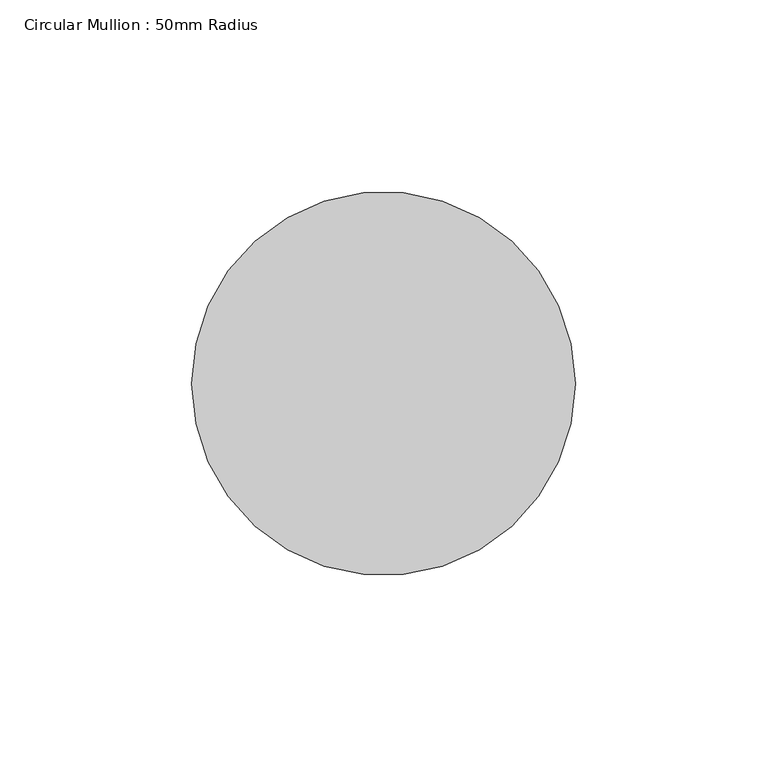
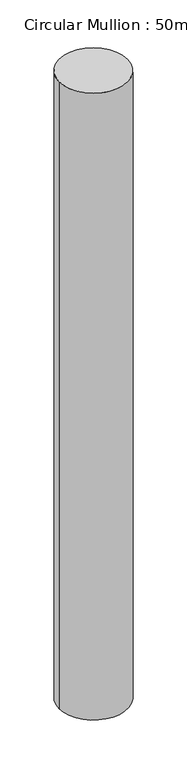
"""IFC4 building model written with IfcOpenShell, lengths in millimetres: member geometry, Circular Mullion : 50mm Radius."""

import ifcopenshell
import ifcopenshell.guid

model = None  # the IFC model being written
_history = None  # IfcOwnerHistory: only IFC2X3 demands one
_inside = {}  # id of a spatial element -> (the spatial element, [elements in it])
_under = {}  # id of a project, library or spatial element -> (it, [spatial elements below it])
_declared = {}  # id of a project -> (the project, [libraries it declares])
_typed = {}  # id of a type object -> (the type object, [elements of that type])
_made_of = {}  # id of a material, layer set ... -> (it, [elements and type objects made of it])


def new_model(schema):
    """Start an empty IFC model of exactly this schema.

    Asked for "IFC4X3", IfcOpenShell would pick the latest addendum, in which some entities
    have other attributes; the version numbers below select the first issue.
    IFC2X3 requires an IfcOwnerHistory on every rooted entity: one is made here for all.
    """
    global model, _history
    if schema == "IFC4X3":
        model = ifcopenshell.file(schema_version=(4, 3, 0, 0))
    else:
        model = ifcopenshell.file(schema=schema)
    _inside.clear()
    _under.clear()
    _declared.clear()
    _typed.clear()
    _made_of.clear()
    _history = None
    if model.schema == "IFC2X3":
        org = make("IfcOrganization", Name="unknown")
        user = make(
            "IfcPersonAndOrganization",
            ThePerson=make("IfcPerson", FamilyName="unknown"),
            TheOrganization=org,
        )
        app = make(
            "IfcApplication",
            ApplicationDeveloper=org,
            Version="unknown",
            ApplicationFullName="unknown",
            ApplicationIdentifier="unknown",
        )
        _history = make(
            "IfcOwnerHistory",
            OwningUser=user,
            OwningApplication=app,
            ChangeAction="ADDED",
            CreationDate=0,
        )
    return model


def make(cls, **values):
    """One entity of the class cls with the attributes given. An attribute that is None is left unset."""
    return model.create_entity(
        cls, **{name: value for name, value in values.items() if value is not None}
    )


def rooted(cls, **values):
    """An entity with a GlobalId (a new one), such as an element, a storey or a relation."""
    return make(cls, GlobalId=ifcopenshell.guid.new(), OwnerHistory=_history, **values)


def si_unit(unit_type, name, prefix=None):
    """IfcSIUnit, for example si_unit("LENGTHUNIT", "METRE", prefix="MILLI")."""
    return make("IfcSIUnit", UnitType=unit_type, Prefix=prefix, Name=name)


def assignment(units):
    """IfcUnitAssignment: the units of a project."""
    return None if units is None else make("IfcUnitAssignment", Units=units)


def point(xyz):
    """IfcCartesianPoint."""
    return None if xyz is None else make("IfcCartesianPoint", Coordinates=xyz)


def direction(xyz):
    """IfcDirection."""
    return None if xyz is None else make("IfcDirection", DirectionRatios=xyz)


def frame(location, z_axis=None, x_axis=None):
    """IfcAxis2Placement3D, a coordinate frame: its origin and axes. An axis left out is left unset."""
    return make(
        "IfcAxis2Placement3D",
        Location=point(location),
        Axis=direction(z_axis),
        RefDirection=direction(x_axis),
    )


def frame_2d(location, x_axis=None):
    """IfcAxis2Placement2D, a coordinate frame in the plane: its origin and x axis."""
    return make(
        "IfcAxis2Placement2D", Location=point(location), RefDirection=direction(x_axis)
    )


def origin():
    """The frame at (0, 0, 0) with its axes left unset."""
    return frame((0.0, 0.0, 0.0))


def origin_2d():
    """The frame at (0, 0) in the plane with its x axis left unset."""
    return frame_2d((0.0, 0.0))


def place(relative_to, where):
    """IfcLocalPlacement: puts the frame where relative to a parent placement (None: the world)."""
    return make(
        "IfcLocalPlacement", PlacementRelTo=relative_to, RelativePlacement=where
    )


def context(
    kind, dimensions, precision=None, world=None, true_north=None, identifier=None
):
    """IfcGeometricRepresentationContext, for example the 3D "Model" context."""
    return make(
        "IfcGeometricRepresentationContext",
        ContextIdentifier=identifier,
        ContextType=kind,
        CoordinateSpaceDimension=dimensions,
        Precision=precision,
        WorldCoordinateSystem=world,
        TrueNorth=true_north,
    )


def project(units=None, contexts=None):
    """IfcProject with its units and contexts."""
    return rooted(
        "IfcProject",
        Name="project",
        RepresentationContexts=contexts,
        UnitsInContext=assignment(units),
    )


def spatial(cls, under=None, at=None, **own):
    """A site, building, storey or space (cls), placed at a placement, below another one or the project."""
    s = rooted(cls, ObjectPlacement=at, **own)
    if under is not None:
        _under.setdefault(under.id(), (under, []))[1].append(s)
    return s


def circle_curve(where, radius):
    """IfcCircle in the frame where."""
    return make("IfcCircle", Position=where, Radius=radius)


def trimmed(basis, trim1, trim2, sense, master):
    """IfcTrimmedCurve: the piece of a basis curve between two trims."""
    return make(
        "IfcTrimmedCurve",
        BasisCurve=basis,
        Trim1=trim1,
        Trim2=trim2,
        SenseAgreement=sense,
        MasterRepresentation=master,
    )


def segment(curve, same_sense, transition):
    """IfcCompositeCurveSegment."""
    return make(
        "IfcCompositeCurveSegment",
        Transition=transition,
        SameSense=same_sense,
        ParentCurve=curve,
    )


def composite_curve(segments, self_intersect=None):
    """IfcCompositeCurve: segments joined end to end."""
    return make("IfcCompositeCurve", Segments=segments, SelfIntersect=self_intersect)


def outline(outer, holes=None, kind="AREA"):
    """IfcArbitraryClosedProfileDef: a profile drawn as a closed curve; with holes, ...WithVoids."""
    if holes is None:
        return make("IfcArbitraryClosedProfileDef", ProfileType=kind, OuterCurve=outer)
    return make(
        "IfcArbitraryProfileDefWithVoids",
        ProfileType=kind,
        OuterCurve=outer,
        InnerCurves=holes,
    )


def extrude(swept, where, along, depth):
    """IfcExtrudedAreaSolid: the profile swept, set in the frame where, extruded along a direction by depth."""
    return make(
        "IfcExtrudedAreaSolid",
        SweptArea=swept,
        Position=where,
        ExtrudedDirection=direction(along),
        Depth=depth,
    )


def shape(context_of_items, identifier, shape_type, items):
    """IfcShapeRepresentation: the items that make up one representation, for example the "Body"."""
    return make(
        "IfcShapeRepresentation",
        ContextOfItems=context_of_items,
        RepresentationIdentifier=identifier,
        RepresentationType=shape_type,
        Items=items,
    )


def source(mapping_origin, context_of_items, identifier, shape_type, items):
    """IfcRepresentationMap: a shape defined once, which mapped items show again and again."""
    return make(
        "IfcRepresentationMap",
        MappingOrigin=mapping_origin,
        MappedRepresentation=shape(context_of_items, identifier, shape_type, items),
    )


def transform(
    local_origin,
    x_axis=None,
    y_axis=None,
    z_axis=None,
    scale=None,
    scale2=None,
    scale3=None,
    uniform=True,
):
    """IfcCartesianTransformationOperator3D, or its non-uniform kind. x_axis, y_axis, z_axis: its Axis1, 2, 3."""
    if uniform:
        return make(
            "IfcCartesianTransformationOperator3D",
            Axis1=direction(x_axis),
            Axis2=direction(y_axis),
            LocalOrigin=point(local_origin),
            Scale=scale,
            Axis3=direction(z_axis),
        )
    return make(
        "IfcCartesianTransformationOperator3DnonUniform",
        Axis1=direction(x_axis),
        Axis2=direction(y_axis),
        LocalOrigin=point(local_origin),
        Scale=scale,
        Axis3=direction(z_axis),
        Scale2=scale2,
        Scale3=scale3,
    )


def mapped(mapping_source, mapping_target):
    """IfcMappedItem: shows the shape of a source again, moved by a transform."""
    return make(
        "IfcMappedItem", MappingSource=mapping_source, MappingTarget=mapping_target
    )


def made_of(thing, what):
    """Note that an element or type object is made of a material, layer set ...; save() writes the relation."""
    if what is not None:
        _made_of.setdefault(what.id(), (what, []))[1].append(thing)
    return thing


def element(
    cls,
    number,
    at=None,
    inside=None,
    cuts=None,
    type_object=None,
    material=None,
    context=None,
    identifier="Body",
    shape_type=None,
    held_by="IfcProductDefinitionShape",
    body=None,
    shapes=None,
    **own,
):
    """One element of the class cls, such as IfcWall. Its Tag is "e" and its number.

    at: its placement. inside: the storey or other place that contains it. cuts: it is an
    opening in that element (IfcRelVoidsElement). A single representation is given by context,
    identifier, shape_type and body (its items); several are given by shapes. held_by: the class
    of the entity that holds the representations. save() writes the other relations.
    """
    e = rooted(cls, Tag="e%d" % number, ObjectPlacement=at, **own)
    if body is not None:
        shapes = [shape(context, identifier, shape_type, body)]
    if shapes is not None:
        e.Representation = make(held_by, Representations=shapes)
    if inside is not None:
        _inside.setdefault(inside.id(), (inside, []))[1].append(e)
    if cuts is not None:
        rooted(
            "IfcRelVoidsElement", RelatingBuildingElement=cuts, RelatedOpeningElement=e
        )
    if type_object is not None:
        _typed.setdefault(type_object.id(), (type_object, []))[1].append(e)
    return made_of(e, material)


def aggregate(whole, parts):
    """IfcRelAggregates: a whole, such as a stair, and the parts it consists of."""
    return rooted("IfcRelAggregates", RelatingObject=whole, RelatedObjects=parts)


def save(model, path):
    """Write the relations noted so far, then the file.

    IfcRelAggregates (storeys below a building ...), IfcRelContainedInSpatialStructure (elements
    in a storey), IfcRelDefinesByType, IfcRelAssociatesMaterial and IfcRelDeclares: one each for
    every whole, place, type object, material and project.
    """
    for whole, parts in _under.values():
        aggregate(whole, parts)
    for where, things in _inside.values():
        rooted(
            "IfcRelContainedInSpatialStructure",
            RelatedElements=things,
            RelatingStructure=where,
        )
    for kind, things in _typed.values():
        rooted("IfcRelDefinesByType", RelatedObjects=things, RelatingType=kind)
    for what, things in _made_of.values():
        rooted("IfcRelAssociatesMaterial", RelatedObjects=things, RelatingMaterial=what)
    for by, libraries in _declared.values():
        rooted("IfcRelDeclares", RelatingContext=by, RelatedDefinitions=libraries)
    model.write(path)


def circular_mullion_50mm_radius_3e5f5aea(model_context):
    return source(origin(), model_context, "Body", "SweptSolid", [
        extrude(outline(composite_curve([segment(trimmed(circle_curve(origin_2d(), 50.0), [point((50.0, 0.0))], [point((-50.0, 0.0))], False, "CARTESIAN"), True, "CONTINUOUS"), segment(trimmed(circle_curve(origin_2d(), 50.0), [point((-50.0, 0.0))], [point((50.0, 0.0))], False, "CARTESIAN"), True, "CONTINUOUS")], self_intersect=False)), frame((0.0, 0.0, -967.5988865), z_axis=(0.0, 0.0, 1.0), x_axis=(1.0, 0.0, 0.0)), (0.0, 0.0, 1.0), 967.5988865),
    ])


if __name__ == "__main__":
    model = new_model("IFC4")
    model_context = context("Model", 3, world=origin())
    ifc_project = project(units=[si_unit("LENGTHUNIT", "METRE", prefix="MILLI")], contexts=[model_context])
    site = spatial("IfcSite", under=ifc_project)
    building = spatial("IfcBuilding", under=site)
    placement = place(None, origin())
    circular_mullion_50mm_radius_shape = circular_mullion_50mm_radius_3e5f5aea(model_context)
    element("IfcMember", 1, ObjectType="Circular Mullion : 50mm Radius", at=placement, inside=building, context=model_context, shape_type="MappedRepresentation", body=[
        mapped(circular_mullion_50mm_radius_shape, transform((0.0, 0.0, 0.0), x_axis=(1.0, 0.0, 0.0), y_axis=(0.0, 1.0, 0.0), z_axis=(0.0, 0.0, 1.0))),
    ])
    save(model, "model.ifc")

# Revit data of these elements
# Type "Circular Mullion : 50mm Radius"
#   built-in parameter 1007350 = 0.164042 (stored number, unit not read)
# Element 1 (IfcMember, "Circular Mullion : 50mm Radius")
#   Materials on its faces: "Aluminium"
# Materials
#   "Aluminium": class "Metal", colour RGB 247 247 247, transparency 0, Description = "Aluminium 6061", Cost = 0
